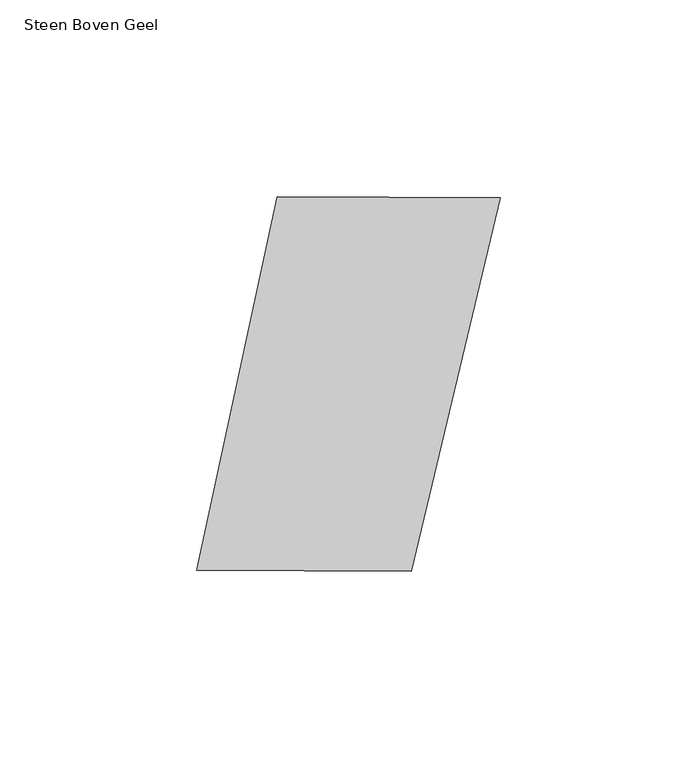
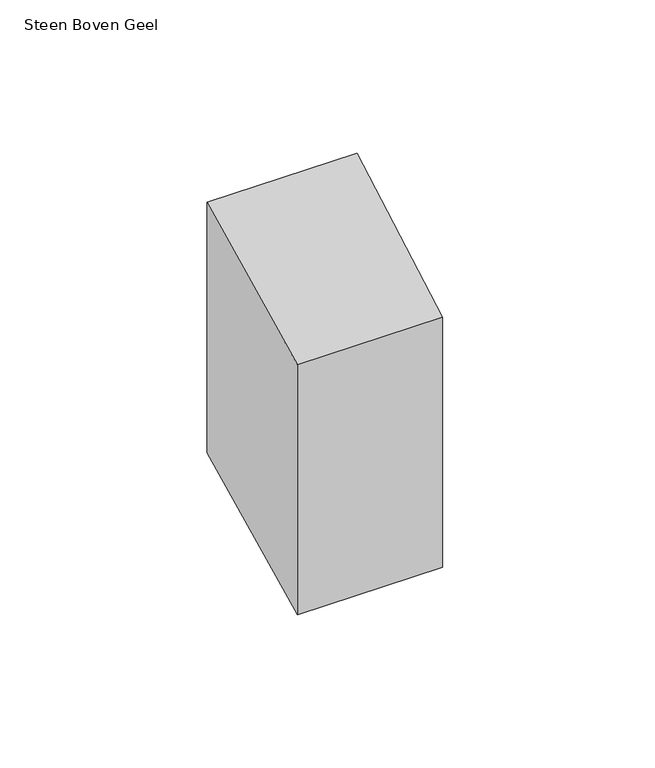
"""IFC4 building model written with IfcOpenShell, lengths in millimetres: proxy geometry, 00_GMA_steen_versie_4 : Steen Boven Geel."""

import ifcopenshell
import ifcopenshell.guid

model = None  # the IFC model being written
_history = None  # IfcOwnerHistory: only IFC2X3 demands one
_inside = {}  # id of a spatial element -> (the spatial element, [elements in it])
_under = {}  # id of a project, library or spatial element -> (it, [spatial elements below it])
_declared = {}  # id of a project -> (the project, [libraries it declares])
_typed = {}  # id of a type object -> (the type object, [elements of that type])
_made_of = {}  # id of a material, layer set ... -> (it, [elements and type objects made of it])


def new_model(schema):
    """Start an empty IFC model of exactly this schema.

    Asked for "IFC4X3", IfcOpenShell would pick the latest addendum, in which some entities
    have other attributes; the version numbers below select the first issue.
    IFC2X3 requires an IfcOwnerHistory on every rooted entity: one is made here for all.
    """
    global model, _history
    if schema == "IFC4X3":
        model = ifcopenshell.file(schema_version=(4, 3, 0, 0))
    else:
        model = ifcopenshell.file(schema=schema)
    _inside.clear()
    _under.clear()
    _declared.clear()
    _typed.clear()
    _made_of.clear()
    _history = None
    if model.schema == "IFC2X3":
        org = make("IfcOrganization", Name="unknown")
        user = make(
            "IfcPersonAndOrganization",
            ThePerson=make("IfcPerson", FamilyName="unknown"),
            TheOrganization=org,
        )
        app = make(
            "IfcApplication",
            ApplicationDeveloper=org,
            Version="unknown",
            ApplicationFullName="unknown",
            ApplicationIdentifier="unknown",
        )
        _history = make(
            "IfcOwnerHistory",
            OwningUser=user,
            OwningApplication=app,
            ChangeAction="ADDED",
            CreationDate=0,
        )
    return model


def make(cls, **values):
    """One entity of the class cls with the attributes given. An attribute that is None is left unset."""
    return model.create_entity(
        cls, **{name: value for name, value in values.items() if value is not None}
    )


def rooted(cls, **values):
    """An entity with a GlobalId (a new one), such as an element, a storey or a relation."""
    return make(cls, GlobalId=ifcopenshell.guid.new(), OwnerHistory=_history, **values)


def si_unit(unit_type, name, prefix=None):
    """IfcSIUnit, for example si_unit("LENGTHUNIT", "METRE", prefix="MILLI")."""
    return make("IfcSIUnit", UnitType=unit_type, Prefix=prefix, Name=name)


def assignment(units):
    """IfcUnitAssignment: the units of a project."""
    return None if units is None else make("IfcUnitAssignment", Units=units)


def point(xyz):
    """IfcCartesianPoint."""
    return None if xyz is None else make("IfcCartesianPoint", Coordinates=xyz)


def direction(xyz):
    """IfcDirection."""
    return None if xyz is None else make("IfcDirection", DirectionRatios=xyz)


def frame(location, z_axis=None, x_axis=None):
    """IfcAxis2Placement3D, a coordinate frame: its origin and axes. An axis left out is left unset."""
    return make(
        "IfcAxis2Placement3D",
        Location=point(location),
        Axis=direction(z_axis),
        RefDirection=direction(x_axis),
    )


def origin():
    """The frame at (0, 0, 0) with its axes left unset."""
    return frame((0.0, 0.0, 0.0))


def origin_with_axes():
    """The frame at (0, 0, 0) with the z axis (0, 0, 1) and the x axis (1, 0, 0) written out."""
    return frame((0.0, 0.0, 0.0), z_axis=(0.0, 0.0, 1.0), x_axis=(1.0, 0.0, 0.0))


def place(relative_to, where):
    """IfcLocalPlacement: puts the frame where relative to a parent placement (None: the world)."""
    return make(
        "IfcLocalPlacement", PlacementRelTo=relative_to, RelativePlacement=where
    )


def context(
    kind, dimensions, precision=None, world=None, true_north=None, identifier=None
):
    """IfcGeometricRepresentationContext, for example the 3D "Model" context."""
    return make(
        "IfcGeometricRepresentationContext",
        ContextIdentifier=identifier,
        ContextType=kind,
        CoordinateSpaceDimension=dimensions,
        Precision=precision,
        WorldCoordinateSystem=world,
        TrueNorth=true_north,
    )


def project(units=None, contexts=None):
    """IfcProject with its units and contexts."""
    return rooted(
        "IfcProject",
        Name="project",
        RepresentationContexts=contexts,
        UnitsInContext=assignment(units),
    )


def spatial(cls, under=None, at=None, **own):
    """A site, building, storey or space (cls), placed at a placement, below another one or the project."""
    s = rooted(cls, ObjectPlacement=at, **own)
    if under is not None:
        _under.setdefault(under.id(), (under, []))[1].append(s)
    return s


def polyline(points):
    """IfcPolyline through the points."""
    return make("IfcPolyline", Points=[point(p) for p in points])


def outline(outer, holes=None, kind="AREA"):
    """IfcArbitraryClosedProfileDef: a profile drawn as a closed curve; with holes, ...WithVoids."""
    if holes is None:
        return make("IfcArbitraryClosedProfileDef", ProfileType=kind, OuterCurve=outer)
    return make(
        "IfcArbitraryProfileDefWithVoids",
        ProfileType=kind,
        OuterCurve=outer,
        InnerCurves=holes,
    )


def extrude(swept, where, along, depth):
    """IfcExtrudedAreaSolid: the profile swept, set in the frame where, extruded along a direction by depth."""
    return make(
        "IfcExtrudedAreaSolid",
        SweptArea=swept,
        Position=where,
        ExtrudedDirection=direction(along),
        Depth=depth,
    )


def shape(context_of_items, identifier, shape_type, items):
    """IfcShapeRepresentation: the items that make up one representation, for example the "Body"."""
    return make(
        "IfcShapeRepresentation",
        ContextOfItems=context_of_items,
        RepresentationIdentifier=identifier,
        RepresentationType=shape_type,
        Items=items,
    )


def source(mapping_origin, context_of_items, identifier, shape_type, items):
    """IfcRepresentationMap: a shape defined once, which mapped items show again and again."""
    return make(
        "IfcRepresentationMap",
        MappingOrigin=mapping_origin,
        MappedRepresentation=shape(context_of_items, identifier, shape_type, items),
    )


def transform(
    local_origin,
    x_axis=None,
    y_axis=None,
    z_axis=None,
    scale=None,
    scale2=None,
    scale3=None,
    uniform=True,
):
    """IfcCartesianTransformationOperator3D, or its non-uniform kind. x_axis, y_axis, z_axis: its Axis1, 2, 3."""
    if uniform:
        return make(
            "IfcCartesianTransformationOperator3D",
            Axis1=direction(x_axis),
            Axis2=direction(y_axis),
            LocalOrigin=point(local_origin),
            Scale=scale,
            Axis3=direction(z_axis),
        )
    return make(
        "IfcCartesianTransformationOperator3DnonUniform",
        Axis1=direction(x_axis),
        Axis2=direction(y_axis),
        LocalOrigin=point(local_origin),
        Scale=scale,
        Axis3=direction(z_axis),
        Scale2=scale2,
        Scale3=scale3,
    )


def mapped(mapping_source, mapping_target):
    """IfcMappedItem: shows the shape of a source again, moved by a transform."""
    return make(
        "IfcMappedItem", MappingSource=mapping_source, MappingTarget=mapping_target
    )


def made_of(thing, what):
    """Note that an element or type object is made of a material, layer set ...; save() writes the relation."""
    if what is not None:
        _made_of.setdefault(what.id(), (what, []))[1].append(thing)
    return thing


def element(
    cls,
    number,
    at=None,
    inside=None,
    cuts=None,
    type_object=None,
    material=None,
    context=None,
    identifier="Body",
    shape_type=None,
    held_by="IfcProductDefinitionShape",
    body=None,
    shapes=None,
    **own,
):
    """One element of the class cls, such as IfcWall. Its Tag is "e" and its number.

    at: its placement. inside: the storey or other place that contains it. cuts: it is an
    opening in that element (IfcRelVoidsElement). A single representation is given by context,
    identifier, shape_type and body (its items); several are given by shapes. held_by: the class
    of the entity that holds the representations. save() writes the other relations.
    """
    e = rooted(cls, Tag="e%d" % number, ObjectPlacement=at, **own)
    if body is not None:
        shapes = [shape(context, identifier, shape_type, body)]
    if shapes is not None:
        e.Representation = make(held_by, Representations=shapes)
    if inside is not None:
        _inside.setdefault(inside.id(), (inside, []))[1].append(e)
    if cuts is not None:
        rooted(
            "IfcRelVoidsElement", RelatingBuildingElement=cuts, RelatedOpeningElement=e
        )
    if type_object is not None:
        _typed.setdefault(type_object.id(), (type_object, []))[1].append(e)
    return made_of(e, material)


def aggregate(whole, parts):
    """IfcRelAggregates: a whole, such as a stair, and the parts it consists of."""
    return rooted("IfcRelAggregates", RelatingObject=whole, RelatedObjects=parts)


def save(model, path):
    """Write the relations noted so far, then the file.

    IfcRelAggregates (storeys below a building ...), IfcRelContainedInSpatialStructure (elements
    in a storey), IfcRelDefinesByType, IfcRelAssociatesMaterial and IfcRelDeclares: one each for
    every whole, place, type object, material and project.
    """
    for whole, parts in _under.values():
        aggregate(whole, parts)
    for where, things in _inside.values():
        rooted(
            "IfcRelContainedInSpatialStructure",
            RelatedElements=things,
            RelatingStructure=where,
        )
    for kind, things in _typed.values():
        rooted("IfcRelDefinesByType", RelatedObjects=things, RelatingType=kind)
    for what, things in _made_of.values():
        rooted("IfcRelAssociatesMaterial", RelatedObjects=things, RelatingMaterial=what)
    for by, libraries in _declared.values():
        rooted("IfcRelDeclares", RelatingContext=by, RelatedDefinitions=libraries)
    model.write(path)


def steen_boven_geel_08aa8c96(model_context):
    return source(origin(), model_context, "Body", "SweptSolid", [
        extrude(outline(polyline([(112.4670872, 118.5627035), (89.7995292, 23.5446719), (35.2524914, 23.833951), (55.8011141, 118.8430583), (112.4670872, 118.5627035)])), origin_with_axes(), (0.0, 0.0, 1.0), 100.0),
    ])


if __name__ == "__main__":
    model = new_model("IFC4")
    model_context = context("Model", 3, world=origin())
    ifc_project = project(units=[si_unit("LENGTHUNIT", "METRE", prefix="MILLI")], contexts=[model_context])
    site = spatial("IfcSite", under=ifc_project)
    building = spatial("IfcBuilding", under=site)
    placement = place(None, origin())
    steen_boven_geel_shape = steen_boven_geel_08aa8c96(model_context)
    element("IfcBuildingElementProxy", 1, Name="00_GMA_steen_versie_4 : Steen Boven Geel", ObjectType="00_GMA_steen_versie_4 : Steen Boven Geel", at=placement, inside=building, context=model_context, shape_type="MappedRepresentation", body=[
        mapped(steen_boven_geel_shape, transform((0.0, 0.0, 0.0), x_axis=(1.0, 0.0, 0.0), y_axis=(0.0, 1.0, 0.0), z_axis=(0.0, 0.0, 1.0))),
    ])
    save(model, "model.ifc")

# Revit data of these elements
# Type "00_GMA_steen_versie_4 : Steen Boven Geel"
#   StootVoegHalfBoven [instance default] = 5 mm
#   StootVoegHalf [instance default] = 5 mm
#   StootVoegBreedteOnder = 10 mm
#   StootVoegBreedteBoven = 10 mm
#   Steendikte = 100 mm
#   LintVoegOnderHalf = 5 mm
#   LintVoegOnder = 10 mm
#   LintVoegBovenHalf = 0 mm
#   LintVoegBoven = 0 mm
#   materiaal = 21_steen_geel
#   MateriaalVoeg = none
#   Default Elevation = 0
# Element 1 (IfcBuildingElementProxy, "00_GMA_steen_versie_4 : Steen Boven Geel")
#   Materials on its faces: "21_steen_geel"
# Materials
#   "21_steen_geel": class "Unassigned", colour RGB 202 202 0, transparency 0, Cost = 0
